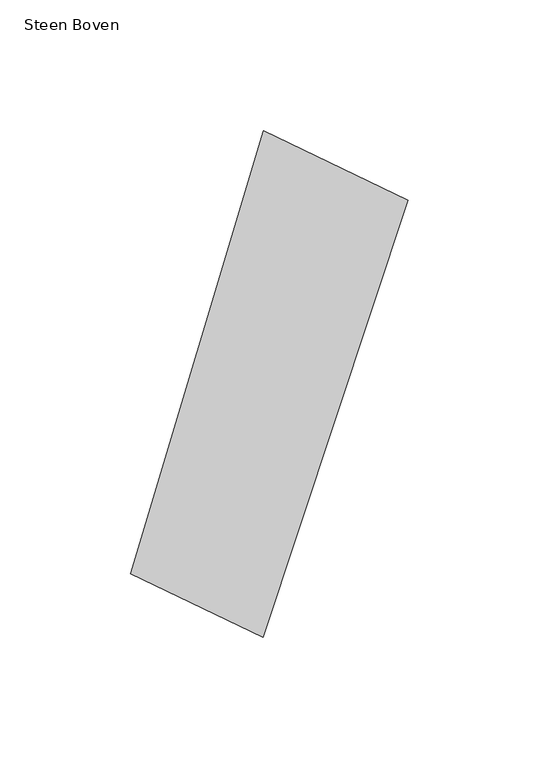
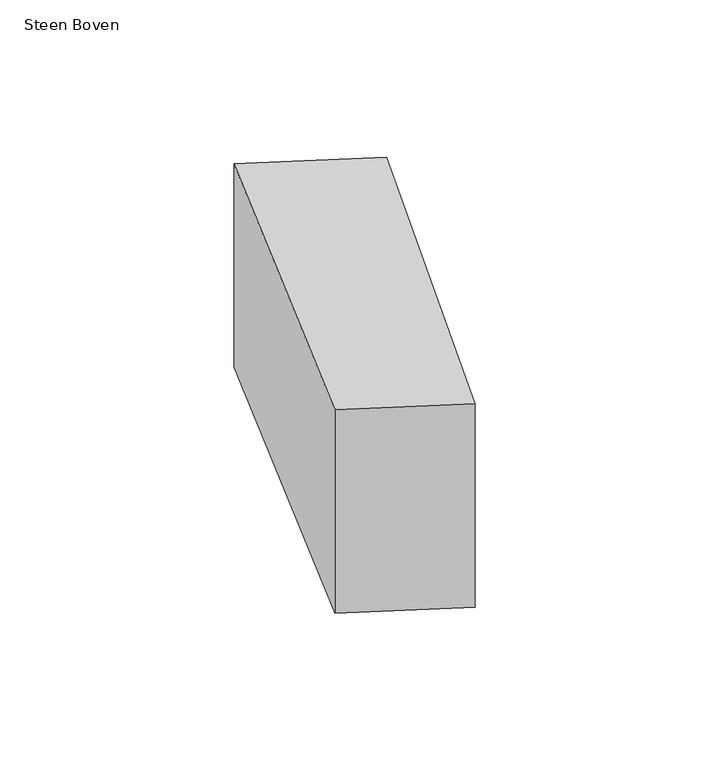
"""IFC4 building model written with IfcOpenShell, lengths in millimetres: proxy geometry, 00_GMA_steen_versie_4 : Steen Boven."""

import ifcopenshell
import ifcopenshell.guid

model = None  # the IFC model being written
_history = None  # IfcOwnerHistory: only IFC2X3 demands one
_inside = {}  # id of a spatial element -> (the spatial element, [elements in it])
_under = {}  # id of a project, library or spatial element -> (it, [spatial elements below it])
_declared = {}  # id of a project -> (the project, [libraries it declares])
_typed = {}  # id of a type object -> (the type object, [elements of that type])
_made_of = {}  # id of a material, layer set ... -> (it, [elements and type objects made of it])


def new_model(schema):
    """Start an empty IFC model of exactly this schema.

    Asked for "IFC4X3", IfcOpenShell would pick the latest addendum, in which some entities
    have other attributes; the version numbers below select the first issue.
    IFC2X3 requires an IfcOwnerHistory on every rooted entity: one is made here for all.
    """
    global model, _history
    if schema == "IFC4X3":
        model = ifcopenshell.file(schema_version=(4, 3, 0, 0))
    else:
        model = ifcopenshell.file(schema=schema)
    _inside.clear()
    _under.clear()
    _declared.clear()
    _typed.clear()
    _made_of.clear()
    _history = None
    if model.schema == "IFC2X3":
        org = make("IfcOrganization", Name="unknown")
        user = make(
            "IfcPersonAndOrganization",
            ThePerson=make("IfcPerson", FamilyName="unknown"),
            TheOrganization=org,
        )
        app = make(
            "IfcApplication",
            ApplicationDeveloper=org,
            Version="unknown",
            ApplicationFullName="unknown",
            ApplicationIdentifier="unknown",
        )
        _history = make(
            "IfcOwnerHistory",
            OwningUser=user,
            OwningApplication=app,
            ChangeAction="ADDED",
            CreationDate=0,
        )
    return model


def make(cls, **values):
    """One entity of the class cls with the attributes given. An attribute that is None is left unset."""
    return model.create_entity(
        cls, **{name: value for name, value in values.items() if value is not None}
    )


def rooted(cls, **values):
    """An entity with a GlobalId (a new one), such as an element, a storey or a relation."""
    return make(cls, GlobalId=ifcopenshell.guid.new(), OwnerHistory=_history, **values)


def si_unit(unit_type, name, prefix=None):
    """IfcSIUnit, for example si_unit("LENGTHUNIT", "METRE", prefix="MILLI")."""
    return make("IfcSIUnit", UnitType=unit_type, Prefix=prefix, Name=name)


def assignment(units):
    """IfcUnitAssignment: the units of a project."""
    return None if units is None else make("IfcUnitAssignment", Units=units)


def point(xyz):
    """IfcCartesianPoint."""
    return None if xyz is None else make("IfcCartesianPoint", Coordinates=xyz)


def direction(xyz):
    """IfcDirection."""
    return None if xyz is None else make("IfcDirection", DirectionRatios=xyz)


def frame(location, z_axis=None, x_axis=None):
    """IfcAxis2Placement3D, a coordinate frame: its origin and axes. An axis left out is left unset."""
    return make(
        "IfcAxis2Placement3D",
        Location=point(location),
        Axis=direction(z_axis),
        RefDirection=direction(x_axis),
    )


def origin():
    """The frame at (0, 0, 0) with its axes left unset."""
    return frame((0.0, 0.0, 0.0))


def origin_with_axes():
    """The frame at (0, 0, 0) with the z axis (0, 0, 1) and the x axis (1, 0, 0) written out."""
    return frame((0.0, 0.0, 0.0), z_axis=(0.0, 0.0, 1.0), x_axis=(1.0, 0.0, 0.0))


def place(relative_to, where):
    """IfcLocalPlacement: puts the frame where relative to a parent placement (None: the world)."""
    return make(
        "IfcLocalPlacement", PlacementRelTo=relative_to, RelativePlacement=where
    )


def context(
    kind, dimensions, precision=None, world=None, true_north=None, identifier=None
):
    """IfcGeometricRepresentationContext, for example the 3D "Model" context."""
    return make(
        "IfcGeometricRepresentationContext",
        ContextIdentifier=identifier,
        ContextType=kind,
        CoordinateSpaceDimension=dimensions,
        Precision=precision,
        WorldCoordinateSystem=world,
        TrueNorth=true_north,
    )


def project(units=None, contexts=None):
    """IfcProject with its units and contexts."""
    return rooted(
        "IfcProject",
        Name="project",
        RepresentationContexts=contexts,
        UnitsInContext=assignment(units),
    )


def spatial(cls, under=None, at=None, **own):
    """A site, building, storey or space (cls), placed at a placement, below another one or the project."""
    s = rooted(cls, ObjectPlacement=at, **own)
    if under is not None:
        _under.setdefault(under.id(), (under, []))[1].append(s)
    return s


def polyline(points):
    """IfcPolyline through the points."""
    return make("IfcPolyline", Points=[point(p) for p in points])


def outline(outer, holes=None, kind="AREA"):
    """IfcArbitraryClosedProfileDef: a profile drawn as a closed curve; with holes, ...WithVoids."""
    if holes is None:
        return make("IfcArbitraryClosedProfileDef", ProfileType=kind, OuterCurve=outer)
    return make(
        "IfcArbitraryProfileDefWithVoids",
        ProfileType=kind,
        OuterCurve=outer,
        InnerCurves=holes,
    )


def extrude(swept, where, along, depth):
    """IfcExtrudedAreaSolid: the profile swept, set in the frame where, extruded along a direction by depth."""
    return make(
        "IfcExtrudedAreaSolid",
        SweptArea=swept,
        Position=where,
        ExtrudedDirection=direction(along),
        Depth=depth,
    )


def shape(context_of_items, identifier, shape_type, items):
    """IfcShapeRepresentation: the items that make up one representation, for example the "Body"."""
    return make(
        "IfcShapeRepresentation",
        ContextOfItems=context_of_items,
        RepresentationIdentifier=identifier,
        RepresentationType=shape_type,
        Items=items,
    )


def source(mapping_origin, context_of_items, identifier, shape_type, items):
    """IfcRepresentationMap: a shape defined once, which mapped items show again and again."""
    return make(
        "IfcRepresentationMap",
        MappingOrigin=mapping_origin,
        MappedRepresentation=shape(context_of_items, identifier, shape_type, items),
    )


def transform(
    local_origin,
    x_axis=None,
    y_axis=None,
    z_axis=None,
    scale=None,
    scale2=None,
    scale3=None,
    uniform=True,
):
    """IfcCartesianTransformationOperator3D, or its non-uniform kind. x_axis, y_axis, z_axis: its Axis1, 2, 3."""
    if uniform:
        return make(
            "IfcCartesianTransformationOperator3D",
            Axis1=direction(x_axis),
            Axis2=direction(y_axis),
            LocalOrigin=point(local_origin),
            Scale=scale,
            Axis3=direction(z_axis),
        )
    return make(
        "IfcCartesianTransformationOperator3DnonUniform",
        Axis1=direction(x_axis),
        Axis2=direction(y_axis),
        LocalOrigin=point(local_origin),
        Scale=scale,
        Axis3=direction(z_axis),
        Scale2=scale2,
        Scale3=scale3,
    )


def mapped(mapping_source, mapping_target):
    """IfcMappedItem: shows the shape of a source again, moved by a transform."""
    return make(
        "IfcMappedItem", MappingSource=mapping_source, MappingTarget=mapping_target
    )


def made_of(thing, what):
    """Note that an element or type object is made of a material, layer set ...; save() writes the relation."""
    if what is not None:
        _made_of.setdefault(what.id(), (what, []))[1].append(thing)
    return thing


def element(
    cls,
    number,
    at=None,
    inside=None,
    cuts=None,
    type_object=None,
    material=None,
    context=None,
    identifier="Body",
    shape_type=None,
    held_by="IfcProductDefinitionShape",
    body=None,
    shapes=None,
    **own,
):
    """One element of the class cls, such as IfcWall. Its Tag is "e" and its number.

    at: its placement. inside: the storey or other place that contains it. cuts: it is an
    opening in that element (IfcRelVoidsElement). A single representation is given by context,
    identifier, shape_type and body (its items); several are given by shapes. held_by: the class
    of the entity that holds the representations. save() writes the other relations.
    """
    e = rooted(cls, Tag="e%d" % number, ObjectPlacement=at, **own)
    if body is not None:
        shapes = [shape(context, identifier, shape_type, body)]
    if shapes is not None:
        e.Representation = make(held_by, Representations=shapes)
    if inside is not None:
        _inside.setdefault(inside.id(), (inside, []))[1].append(e)
    if cuts is not None:
        rooted(
            "IfcRelVoidsElement", RelatingBuildingElement=cuts, RelatedOpeningElement=e
        )
    if type_object is not None:
        _typed.setdefault(type_object.id(), (type_object, []))[1].append(e)
    return made_of(e, material)


def aggregate(whole, parts):
    """IfcRelAggregates: a whole, such as a stair, and the parts it consists of."""
    return rooted("IfcRelAggregates", RelatingObject=whole, RelatedObjects=parts)


def save(model, path):
    """Write the relations noted so far, then the file.

    IfcRelAggregates (storeys below a building ...), IfcRelContainedInSpatialStructure (elements
    in a storey), IfcRelDefinesByType, IfcRelAssociatesMaterial and IfcRelDeclares: one each for
    every whole, place, type object, material and project.
    """
    for whole, parts in _under.values():
        aggregate(whole, parts)
    for where, things in _inside.values():
        rooted(
            "IfcRelContainedInSpatialStructure",
            RelatedElements=things,
            RelatingStructure=where,
        )
    for kind, things in _typed.values():
        rooted("IfcRelDefinesByType", RelatedObjects=things, RelatingType=kind)
    for what, things in _made_of.values():
        rooted("IfcRelAssociatesMaterial", RelatedObjects=things, RelatingMaterial=what)
    for by, libraries in _declared.values():
        rooted("IfcRelDeclares", RelatingContext=by, RelatedDefinitions=libraries)
    model.write(path)


def steen_boven_d55e3ff2(model_context):
    return source(origin(), model_context, "Body", "SweptSolid", [
        extrude(outline(polyline([(129.6260275, 156.8862065), (74.0423779, -10.6153003), (23.1857256, 13.8244684), (74.2668272, 183.5100366), (129.6260275, 156.8862065)])), origin_with_axes(), (0.0, 0.0, 1.0), 100.0),
    ])


if __name__ == "__main__":
    model = new_model("IFC4")
    model_context = context("Model", 3, world=origin())
    ifc_project = project(units=[si_unit("LENGTHUNIT", "METRE", prefix="MILLI")], contexts=[model_context])
    site = spatial("IfcSite", under=ifc_project)
    building = spatial("IfcBuilding", under=site)
    placement = place(None, origin())
    steen_boven_shape = steen_boven_d55e3ff2(model_context)
    element("IfcBuildingElementProxy", 1, Name="00_GMA_steen_versie_4 : Steen Boven", ObjectType="00_GMA_steen_versie_4 : Steen Boven", at=placement, inside=building, context=model_context, shape_type="MappedRepresentation", body=[
        mapped(steen_boven_shape, transform((0.0, 0.0, 0.0), x_axis=(1.0, 0.0, 0.0), y_axis=(0.0, 1.0, 0.0), z_axis=(0.0, 0.0, 1.0))),
    ])
    save(model, "model.ifc")

# Revit data of these elements
# Type "00_GMA_steen_versie_4 : Steen Boven"
#   StootVoegHalfBoven [instance default] = 5 mm
#   StootVoegHalf [instance default] = 5 mm
#   StootVoegBreedteOnder = 10 mm
#   StootVoegBreedteBoven = 10 mm
#   Steendikte = 100 mm
#   LintVoegOnderHalf = 5 mm
#   LintVoegOnder = 10 mm
#   LintVoegBovenHalf = 0 mm
#   LintVoegBoven = 0 mm
#   materiaal = none
#   MateriaalVoeg = none
#   Default Elevation = 0
